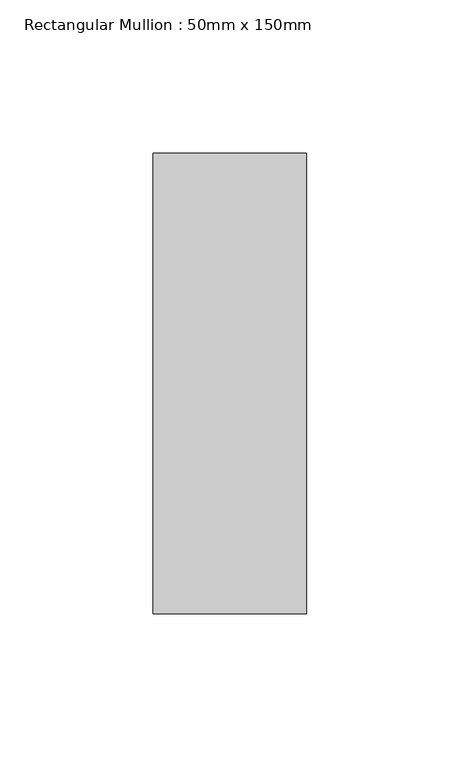
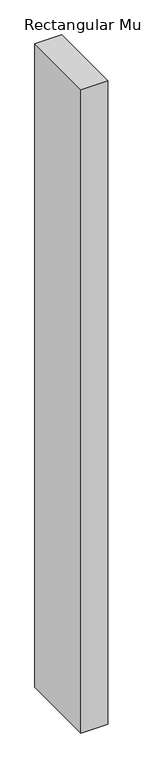
"""IFC4 building model written with IfcOpenShell, lengths in millimetres: member geometry, Rectangular Mullion : 50mm x 150mm."""

import ifcopenshell
import ifcopenshell.guid

model = None  # the IFC model being written
_history = None  # IfcOwnerHistory: only IFC2X3 demands one
_inside = {}  # id of a spatial element -> (the spatial element, [elements in it])
_under = {}  # id of a project, library or spatial element -> (it, [spatial elements below it])
_declared = {}  # id of a project -> (the project, [libraries it declares])
_typed = {}  # id of a type object -> (the type object, [elements of that type])
_made_of = {}  # id of a material, layer set ... -> (it, [elements and type objects made of it])


def new_model(schema):
    """Start an empty IFC model of exactly this schema.

    Asked for "IFC4X3", IfcOpenShell would pick the latest addendum, in which some entities
    have other attributes; the version numbers below select the first issue.
    IFC2X3 requires an IfcOwnerHistory on every rooted entity: one is made here for all.
    """
    global model, _history
    if schema == "IFC4X3":
        model = ifcopenshell.file(schema_version=(4, 3, 0, 0))
    else:
        model = ifcopenshell.file(schema=schema)
    _inside.clear()
    _under.clear()
    _declared.clear()
    _typed.clear()
    _made_of.clear()
    _history = None
    if model.schema == "IFC2X3":
        org = make("IfcOrganization", Name="unknown")
        user = make(
            "IfcPersonAndOrganization",
            ThePerson=make("IfcPerson", FamilyName="unknown"),
            TheOrganization=org,
        )
        app = make(
            "IfcApplication",
            ApplicationDeveloper=org,
            Version="unknown",
            ApplicationFullName="unknown",
            ApplicationIdentifier="unknown",
        )
        _history = make(
            "IfcOwnerHistory",
            OwningUser=user,
            OwningApplication=app,
            ChangeAction="ADDED",
            CreationDate=0,
        )
    return model


def make(cls, **values):
    """One entity of the class cls with the attributes given. An attribute that is None is left unset."""
    return model.create_entity(
        cls, **{name: value for name, value in values.items() if value is not None}
    )


def rooted(cls, **values):
    """An entity with a GlobalId (a new one), such as an element, a storey or a relation."""
    return make(cls, GlobalId=ifcopenshell.guid.new(), OwnerHistory=_history, **values)


def si_unit(unit_type, name, prefix=None):
    """IfcSIUnit, for example si_unit("LENGTHUNIT", "METRE", prefix="MILLI")."""
    return make("IfcSIUnit", UnitType=unit_type, Prefix=prefix, Name=name)


def assignment(units):
    """IfcUnitAssignment: the units of a project."""
    return None if units is None else make("IfcUnitAssignment", Units=units)


def point(xyz):
    """IfcCartesianPoint."""
    return None if xyz is None else make("IfcCartesianPoint", Coordinates=xyz)


def direction(xyz):
    """IfcDirection."""
    return None if xyz is None else make("IfcDirection", DirectionRatios=xyz)


def frame(location, z_axis=None, x_axis=None):
    """IfcAxis2Placement3D, a coordinate frame: its origin and axes. An axis left out is left unset."""
    return make(
        "IfcAxis2Placement3D",
        Location=point(location),
        Axis=direction(z_axis),
        RefDirection=direction(x_axis),
    )


def origin():
    """The frame at (0, 0, 0) with its axes left unset."""
    return frame((0.0, 0.0, 0.0))


def place(relative_to, where):
    """IfcLocalPlacement: puts the frame where relative to a parent placement (None: the world)."""
    return make(
        "IfcLocalPlacement", PlacementRelTo=relative_to, RelativePlacement=where
    )


def context(
    kind, dimensions, precision=None, world=None, true_north=None, identifier=None
):
    """IfcGeometricRepresentationContext, for example the 3D "Model" context."""
    return make(
        "IfcGeometricRepresentationContext",
        ContextIdentifier=identifier,
        ContextType=kind,
        CoordinateSpaceDimension=dimensions,
        Precision=precision,
        WorldCoordinateSystem=world,
        TrueNorth=true_north,
    )


def project(units=None, contexts=None):
    """IfcProject with its units and contexts."""
    return rooted(
        "IfcProject",
        Name="project",
        RepresentationContexts=contexts,
        UnitsInContext=assignment(units),
    )


def spatial(cls, under=None, at=None, **own):
    """A site, building, storey or space (cls), placed at a placement, below another one or the project."""
    s = rooted(cls, ObjectPlacement=at, **own)
    if under is not None:
        _under.setdefault(under.id(), (under, []))[1].append(s)
    return s


def polyline(points):
    """IfcPolyline through the points."""
    return make("IfcPolyline", Points=[point(p) for p in points])


def outline(outer, holes=None, kind="AREA"):
    """IfcArbitraryClosedProfileDef: a profile drawn as a closed curve; with holes, ...WithVoids."""
    if holes is None:
        return make("IfcArbitraryClosedProfileDef", ProfileType=kind, OuterCurve=outer)
    return make(
        "IfcArbitraryProfileDefWithVoids",
        ProfileType=kind,
        OuterCurve=outer,
        InnerCurves=holes,
    )


def extrude(swept, where, along, depth):
    """IfcExtrudedAreaSolid: the profile swept, set in the frame where, extruded along a direction by depth."""
    return make(
        "IfcExtrudedAreaSolid",
        SweptArea=swept,
        Position=where,
        ExtrudedDirection=direction(along),
        Depth=depth,
    )


def shape(context_of_items, identifier, shape_type, items):
    """IfcShapeRepresentation: the items that make up one representation, for example the "Body"."""
    return make(
        "IfcShapeRepresentation",
        ContextOfItems=context_of_items,
        RepresentationIdentifier=identifier,
        RepresentationType=shape_type,
        Items=items,
    )


def source(mapping_origin, context_of_items, identifier, shape_type, items):
    """IfcRepresentationMap: a shape defined once, which mapped items show again and again."""
    return make(
        "IfcRepresentationMap",
        MappingOrigin=mapping_origin,
        MappedRepresentation=shape(context_of_items, identifier, shape_type, items),
    )


def transform(
    local_origin,
    x_axis=None,
    y_axis=None,
    z_axis=None,
    scale=None,
    scale2=None,
    scale3=None,
    uniform=True,
):
    """IfcCartesianTransformationOperator3D, or its non-uniform kind. x_axis, y_axis, z_axis: its Axis1, 2, 3."""
    if uniform:
        return make(
            "IfcCartesianTransformationOperator3D",
            Axis1=direction(x_axis),
            Axis2=direction(y_axis),
            LocalOrigin=point(local_origin),
            Scale=scale,
            Axis3=direction(z_axis),
        )
    return make(
        "IfcCartesianTransformationOperator3DnonUniform",
        Axis1=direction(x_axis),
        Axis2=direction(y_axis),
        LocalOrigin=point(local_origin),
        Scale=scale,
        Axis3=direction(z_axis),
        Scale2=scale2,
        Scale3=scale3,
    )


def mapped(mapping_source, mapping_target):
    """IfcMappedItem: shows the shape of a source again, moved by a transform."""
    return make(
        "IfcMappedItem", MappingSource=mapping_source, MappingTarget=mapping_target
    )


def made_of(thing, what):
    """Note that an element or type object is made of a material, layer set ...; save() writes the relation."""
    if what is not None:
        _made_of.setdefault(what.id(), (what, []))[1].append(thing)
    return thing


def element(
    cls,
    number,
    at=None,
    inside=None,
    cuts=None,
    type_object=None,
    material=None,
    context=None,
    identifier="Body",
    shape_type=None,
    held_by="IfcProductDefinitionShape",
    body=None,
    shapes=None,
    **own,
):
    """One element of the class cls, such as IfcWall. Its Tag is "e" and its number.

    at: its placement. inside: the storey or other place that contains it. cuts: it is an
    opening in that element (IfcRelVoidsElement). A single representation is given by context,
    identifier, shape_type and body (its items); several are given by shapes. held_by: the class
    of the entity that holds the representations. save() writes the other relations.
    """
    e = rooted(cls, Tag="e%d" % number, ObjectPlacement=at, **own)
    if body is not None:
        shapes = [shape(context, identifier, shape_type, body)]
    if shapes is not None:
        e.Representation = make(held_by, Representations=shapes)
    if inside is not None:
        _inside.setdefault(inside.id(), (inside, []))[1].append(e)
    if cuts is not None:
        rooted(
            "IfcRelVoidsElement", RelatingBuildingElement=cuts, RelatedOpeningElement=e
        )
    if type_object is not None:
        _typed.setdefault(type_object.id(), (type_object, []))[1].append(e)
    return made_of(e, material)


def aggregate(whole, parts):
    """IfcRelAggregates: a whole, such as a stair, and the parts it consists of."""
    return rooted("IfcRelAggregates", RelatingObject=whole, RelatedObjects=parts)


def save(model, path):
    """Write the relations noted so far, then the file.

    IfcRelAggregates (storeys below a building ...), IfcRelContainedInSpatialStructure (elements
    in a storey), IfcRelDefinesByType, IfcRelAssociatesMaterial and IfcRelDeclares: one each for
    every whole, place, type object, material and project.
    """
    for whole, parts in _under.values():
        aggregate(whole, parts)
    for where, things in _inside.values():
        rooted(
            "IfcRelContainedInSpatialStructure",
            RelatedElements=things,
            RelatingStructure=where,
        )
    for kind, things in _typed.values():
        rooted("IfcRelDefinesByType", RelatedObjects=things, RelatingType=kind)
    for what, things in _made_of.values():
        rooted("IfcRelAssociatesMaterial", RelatedObjects=things, RelatingMaterial=what)
    for by, libraries in _declared.values():
        rooted("IfcRelDeclares", RelatingContext=by, RelatedDefinitions=libraries)
    model.write(path)


def rectangular_mullion_50mm_x_150mm_11a5ee59(model_context):
    return source(origin(), model_context, "Body", "SweptSolid", [
        extrude(outline(polyline([(0.0, 75.0), (0.0, -75.0), (-50.0, -75.0), (-50.0, 75.0), (0.0, 75.0)])), frame((0.0, 0.0, -1278.5714285), z_axis=(0.0, 0.0, 1.0), x_axis=(1.0, 0.0, 0.0)), (0.0, 0.0, 1.0), 1278.5714285),
    ])


if __name__ == "__main__":
    model = new_model("IFC4")
    model_context = context("Model", 3, world=origin())
    ifc_project = project(units=[si_unit("LENGTHUNIT", "METRE", prefix="MILLI")], contexts=[model_context])
    site = spatial("IfcSite", under=ifc_project)
    building = spatial("IfcBuilding", under=site)
    placement = place(None, origin())
    rectangular_mullion_50mm_x_150mm_shape = rectangular_mullion_50mm_x_150mm_11a5ee59(model_context)
    element("IfcMember", 1, ObjectType="Rectangular Mullion : 50mm x 150mm", at=placement, inside=building, context=model_context, shape_type="MappedRepresentation", body=[
        mapped(rectangular_mullion_50mm_x_150mm_shape, transform((0.0, 0.0, 0.0), x_axis=(1.0, 0.0, 0.0), y_axis=(0.0, 1.0, 0.0), z_axis=(0.0, 0.0, 1.0))),
    ])
    save(model, "model.ifc")

# Revit data of these elements
# Type "Rectangular Mullion : 50mm x 150mm"
#   built-in parameter 1007304 = 0.492126 (stored number, unit not read)
#   built-in parameter 1007301 = 0.082021 (stored number, unit not read)
#   built-in parameter 1007300 = 0.082021 (stored number, unit not read)
# Element 1 (IfcMember, "Rectangular Mullion : 50mm x 150mm")
#   Materials on its faces: "Aluminum"
# Materials
#   "Aluminum": class "Metal", colour RGB 247 247 247, transparency 0, Description = "Aluminum 6061", Cost = 0
